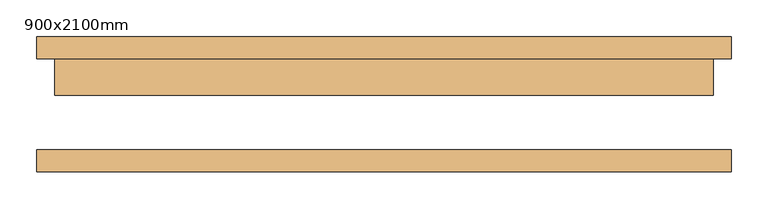
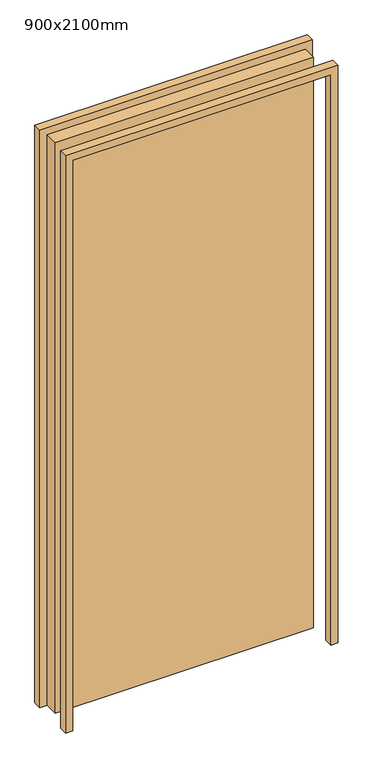
"""IFC4 building model written with IfcOpenShell, lengths in millimetres: door geometry, WWm-SingleSolid-Flush : 900x2100mm."""

from ifc_helpers import new_model, si_unit, frame, origin, origin_with_axes, place, context, project, spatial, polyline, outline, extrude, source, transform, mapped, element, save


def door_900x2100mm_3c828951(model_context):
    return source(origin(), model_context, "Body", "SweptSolid", [
        extrude(outline(polyline([(2125.0, -475.0), (0.0, -475.0), (0.0, -450.0), (2100.0, -450.0), (2100.0, 450.0), (0.0, 450.0), (0.0, 475.0), (2125.0, 475.0), (2125.0, -475.0)])), frame((0.0, 62.5, 0.0), z_axis=(0.0, 1.0, 0.0), x_axis=(0.0, 0.0, 1.0)), (0.0, 0.0, 1.0), 30.0),
        extrude(outline(polyline([(2125.0, 475.0), (2125.0, -475.0), (0.0, -475.0), (0.0, -450.0), (2100.0, -450.0), (2100.0, 450.0), (0.0, 450.0), (0.0, 475.0), (2125.0, 475.0)])), frame((0.0, -92.5, 0.0), z_axis=(0.0, 1.0, 0.0), x_axis=(0.0, 0.0, 1.0)), (0.0, 0.0, 1.0), 30.0),
        extrude(outline(polyline([(450.0, 12.5), (-450.0, 12.5), (-450.0, 62.5), (450.0, 62.5), (450.0, 12.5)])), origin_with_axes(), (0.0, 0.0, 1.0), 2100.0),
    ])


if __name__ == "__main__":
    model = new_model("IFC4")
    model_context = context("Model", 3, world=origin())
    ifc_project = project(units=[si_unit("LENGTHUNIT", "METRE", prefix="MILLI")], contexts=[model_context])
    site = spatial("IfcSite", under=ifc_project)
    building = spatial("IfcBuilding", under=site)
    placement = place(None, origin())
    door_900x2100mm_shape = door_900x2100mm_3c828951(model_context)
    element("IfcDoor", 1, ObjectType="WWm-SingleSolid-Flush : 900x2100mm", at=placement, inside=building, context=model_context, shape_type="MappedRepresentation", body=[
        mapped(door_900x2100mm_shape, transform((0.0, 0.0, 0.0), x_axis=(1.0, 0.0, 0.0), y_axis=(0.0, 1.0, 0.0), z_axis=(0.0, 0.0, 1.0))),
    ])
    save(model, "model.ifc")

# Revit data of these elements
# Type "WWm-SingleSolid-Flush : 900x2100mm"
#   Type Mark = "EX1-52"
#   Construction Type Id = "MDOOR"
#   Assembly Code = "C1020"
#   Analytic Construction = "Metal"
#   Thickness = 50 mm
#   Thermal Resistance (R) = 0.270117 (m²·K)/W
#   Heat Transfer Coefficient (U) = 3.7021 W/(m²·K)
#   Height = 2100 mm
#   Trim Projection Ext = 30 mm
#   Trim Projection Int = 30 mm
#   Trim Width = 25 mm
#   Width = 900 mm
#   Not 90 Degree [instance default] = no
#   90 Degree [instance default] = yes
#   Door Material = WW-EC-RGB-White
#   Frame Material = WW-EC-RGB-White
#   Visual Light Transmittance = 0
#   Solar Heat Gain Coefficient = 0
#   Function = (empty or 0)
#   Wall Closure = (empty or 0)
# Element 1 (IfcDoor, "WWm-SingleSolid-Flush : 900x2100mm")
#   Materials on its faces: "WW-EC-RGB-White"
# Materials
#   "WW-EC-RGB-White": class "Generic", colour RGB 255 255 255, transparency 0, Comments = "If region requests off-white, swith asset color to RGB 231-228-220", Description = "Generic Color", Cost = 0
